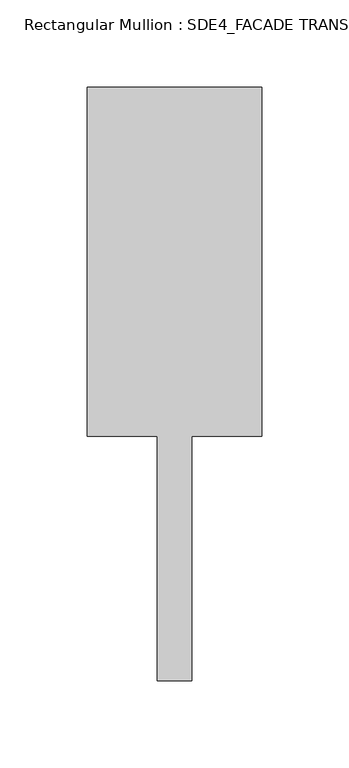
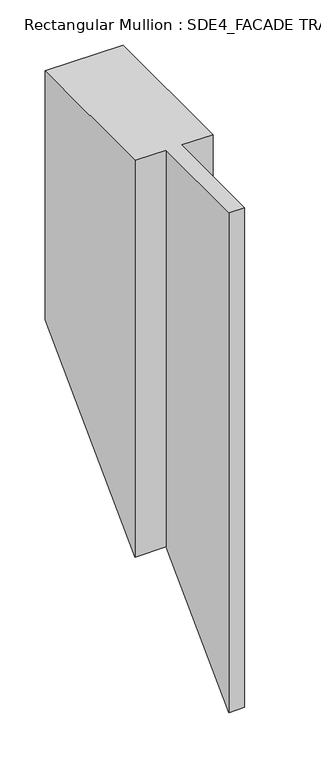
"""IFC4 building model written with IfcOpenShell, lengths in millimetres: member geometry, Rectangular Mullion : SDE4_FACADE TRANSOM TYPE 1."""

from ifc_helpers import new_model, si_unit, origin, place, context, project, spatial, faceted_brep, source, transform, mapped, element, save


def rectangular_mullion_sde4_facade_transom_type_1_ac9d8054(model_context):
    return source(origin(), model_context, "Body", "Brep", [
        faceted_brep([(50.0, 132.5, 0.0), (-50.0, 132.5, 0.0), (-50.0, -67.5, 0.0), (-10.0, -67.5, 0.0), (-10.0, -207.5, 0.0), (10.0, -207.5, 0.0), (10.0, -67.5, 0.0), (50.0, -67.5, 0.0), (50.0, 132.5, -337.5), (-50.0, 132.5, -337.5), (-50.0, -67.5, -537.5), (-10.0, -67.5, -537.5), (-10.0, -207.5, -677.5), (10.0, -207.5, -677.5), (10.0, -67.5, -537.5), (50.0, -67.5, -537.5)], [[[0, 1, 2, 3, 4, 5, 6, 7]], [[1, 0, 8, 9]], [[2, 1, 9, 10]], [[3, 2, 10, 11]], [[4, 3, 11, 12]], [[5, 4, 12, 13]], [[6, 5, 13, 14]], [[7, 6, 14, 15]], [[0, 7, 15, 8]], [[8, 15, 14, 13, 12, 11, 10, 9]]]),
    ])


if __name__ == "__main__":
    model = new_model("IFC4")
    model_context = context("Model", 3, world=origin())
    ifc_project = project(units=[si_unit("LENGTHUNIT", "METRE", prefix="MILLI")], contexts=[model_context])
    site = spatial("IfcSite", under=ifc_project)
    building = spatial("IfcBuilding", under=site)
    placement = place(None, origin())
    rectangular_mullion_sde4_facade_transom_type_1_shape = rectangular_mullion_sde4_facade_transom_type_1_ac9d8054(model_context)
    element("IfcMember", 1, ObjectType="Rectangular Mullion : SDE4_FACADE TRANSOM TYPE 1", at=placement, inside=building, context=model_context, shape_type="MappedRepresentation", body=[
        mapped(rectangular_mullion_sde4_facade_transom_type_1_shape, transform((0.0, 0.0, 0.0), x_axis=(1.0, 0.0, 0.0), y_axis=(0.0, 1.0, 0.0), z_axis=(0.0, 0.0, 1.0))),
    ])
    save(model, "model.ifc")

# Revit data of these elements
# Type "Rectangular Mullion : SDE4_FACADE TRANSOM TYPE 1"
#   built-in parameter 1007322 = 1.11549 (stored number, unit not read)
#   built-in parameter 1007321 = 0.164042 (stored number, unit not read)
#   built-in parameter 1007320 = 0.164042 (stored number, unit not read)
